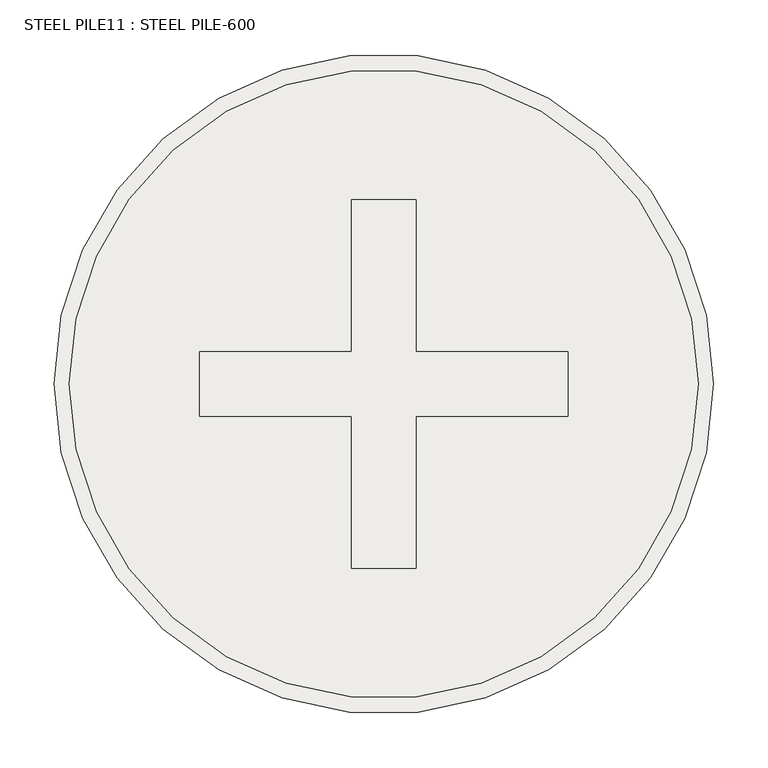
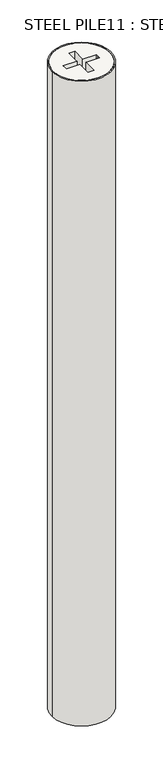
"""IFC4 building model written with IfcOpenShell, lengths in millimetres: slab geometry, STEEL PILE11 : STEEL PILE-600."""

from ifc_helpers import new_model, si_unit, point, frame, frame_2d, origin, place, context, project, spatial, circle_curve, trimmed, segment, composite_curve, outline, extrude, source, transform, mapped, element, save
from ifc_brep_helpers import plane_surface, cylinder_surface, advanced_brep


def steel_pile11_steel_pile_600_0914329d(model_context):
    return source(origin(), model_context, "Body", "SolidModel", [
        advanced_brep(
        [(5709.5, 25499.5208589, 150.0), (6290.5, 25499.5208589, 150.0), (5970.0, 25469.5208589, 150.0), (5830.0, 25469.5208589, 150.0), (5830.0, 25499.5208589, 150.0), (5830.0, 25529.5208589, 150.0), (5970.0, 25529.5208589, 150.0), (5970.0, 25669.5208589, 150.0), (6030.0, 25669.5208589, 150.0), (6030.0, 25529.5208589, 150.0), (6170.0, 25529.5208589, 150.0), (6170.0, 25499.5208589, 150.0), (6170.0, 25469.5208589, 150.0), (6030.0, 25469.5208589, 150.0), (6030.0, 25329.5208589, 150.0), (5970.0, 25329.5208589, 150.0), (5709.5, 25499.5208589, -1850.0), (6290.5, 25499.5208589, -1850.0), (5830.0, 25469.5208589, -160.0), (5970.0, 25469.5208589, -160.0), (5970.0, 25329.5208589, -160.0), (6030.0, 25329.5208589, -160.0), (6030.0, 25469.5208589, -160.0), (6170.0, 25469.5208589, -160.0), (6170.0, 25499.5208589, -160.0), (6170.0, 25529.5208589, -160.0), (6030.0, 25529.5208589, -160.0), (6030.0, 25669.5208589, -160.0), (5970.0, 25669.5208589, -160.0), (5970.0, 25529.5208589, -160.0), (5830.0, 25529.5208589, -160.0), (5830.0, 25499.5208589, -160.0)],
        [
            (0, 1, circle_curve(frame((6000.0, 25499.5208589, 150.0), z_axis=(0.0, 0.0, 1.0), x_axis=(1.0, 0.0, 0.0)), 290.5)),
            (1, 0, circle_curve(frame((6000.0, 25499.5208589, 150.0), z_axis=(0.0, 0.0, 1.0), x_axis=(1.0, 0.0, 0.0)), 290.5)),
            (2, 3),
            (3, 4),
            (4, 5),
            (5, 6),
            (6, 7),
            (7, 8),
            (8, 9),
            (9, 10),
            (10, 11),
            (11, 12),
            (12, 13),
            (13, 14),
            (14, 15),
            (15, 2),
            (16, 17, circle_curve(frame((6000.0, 25499.5208589, -1850.0), z_axis=(0.0, 0.0, -1.0), x_axis=(1.0, 0.0, 0.0)), 290.5)),
            (17, 16, circle_curve(frame((6000.0, 25499.5208589, -1850.0), z_axis=(0.0, 0.0, -1.0), x_axis=(1.0, 0.0, 0.0)), 290.5)),
            (0, 16),
            (17, 1),
            (18, 19),
            (19, 20),
            (20, 21),
            (21, 22),
            (22, 23),
            (23, 24),
            (24, 25),
            (25, 26),
            (26, 27),
            (27, 28),
            (28, 29),
            (29, 30),
            (30, 31),
            (31, 18),
            (18, 3),
            (2, 19),
            (15, 20),
            (14, 21),
            (13, 22),
            (12, 23),
            (11, 24),
            (10, 25),
            (9, 26),
            (8, 27),
            (7, 28),
            (6, 29),
            (5, 30),
            (4, 31),
        ],
        [
            plane_surface(frame((6290.5, 25499.5208589, 150.0), z_axis=(0.0, 0.0, 1.0), x_axis=(0.0, 1.0, 0.0))),
            plane_surface(frame((6290.5, 25499.5208589, -1850.0), z_axis=(0.0, 0.0, -1.0), x_axis=(0.0, -1.0, 0.0))),
            cylinder_surface(frame((6000.0, 25499.5208589, -1850.0), z_axis=(0.0, 0.0, 1.0), x_axis=(1.0, 0.0, 0.0)), 290.5),
            plane_surface(frame((5830.0, 25469.5208589, -160.0), z_axis=(0.0, 0.0, 1.0), x_axis=(-1.0, 0.0, 0.0))),
            plane_surface(frame((5830.0, 25469.5208589, 160.0), z_axis=(0.0, 1.0, 0.0), x_axis=(0.0, 0.0, -1.0))),
            plane_surface(frame((5970.0, 25469.5208589, 160.0), z_axis=(1.0, 0.0, 0.0), x_axis=(0.0, 0.0, -1.0))),
            plane_surface(frame((5970.0, 25329.5208589, 160.0), z_axis=(0.0, 1.0, 0.0), x_axis=(0.0, 0.0, -1.0))),
            plane_surface(frame((6030.0, 25329.5208589, 160.0), z_axis=(-1.0, 0.0, 0.0), x_axis=(0.0, 0.0, -1.0))),
            plane_surface(frame((6030.0, 25469.5208589, 160.0), z_axis=(0.0, 1.0, 0.0), x_axis=(0.0, 0.0, -1.0))),
            plane_surface(frame((6170.0, 25469.5208589, 160.0), z_axis=(-1.0, 0.0, 0.0), x_axis=(0.0, 0.0, -1.0))),
            plane_surface(frame((6170.0, 25499.5208589, 160.0), z_axis=(-1.0, 0.0, 0.0), x_axis=(0.0, 0.0, -1.0))),
            plane_surface(frame((6170.0, 25529.5208589, 160.0), z_axis=(0.0, -1.0, 0.0), x_axis=(0.0, 0.0, -1.0))),
            plane_surface(frame((6030.0, 25529.5208589, 160.0), z_axis=(-1.0, 0.0, 0.0), x_axis=(0.0, 0.0, -1.0))),
            plane_surface(frame((6030.0, 25669.5208589, 160.0), z_axis=(0.0, -1.0, 0.0), x_axis=(0.0, 0.0, -1.0))),
            plane_surface(frame((5970.0, 25669.5208589, 160.0), z_axis=(1.0, 0.0, 0.0), x_axis=(0.0, 0.0, -1.0))),
            plane_surface(frame((5970.0, 25529.5208589, 160.0), z_axis=(0.0, -1.0, 0.0), x_axis=(0.0, 0.0, -1.0))),
            plane_surface(frame((5830.0, 25529.5208589, 160.0), z_axis=(1.0, 0.0, 0.0), x_axis=(0.0, 0.0, -1.0))),
            plane_surface(frame((5830.0, 25499.5208589, 160.0), z_axis=(1.0, 0.0, 0.0), x_axis=(0.0, 0.0, -1.0))),
        ],
        [
            (0, [[1, 2], [3, 4, 5, 6, 7, 8, 9, 10, 11, 12, 13, 14, 15, 16]]),
            (1, [[17, 18]]),
            (2, [[-1, 19, -18, 20]]),
            (2, [[-2, -20, -17, -19]]),
            (3, [[21, 22, 23, 24, 25, 26, 27, 28, 29, 30, 31, 32, 33, 34]]),
            (4, [[-21, 35, -3, 36]]),
            (5, [[-22, -36, -16, 37]]),
            (6, [[-23, -37, -15, 38]]),
            (7, [[-24, -38, -14, 39]]),
            (8, [[-25, -39, -13, 40]]),
            (9, [[-26, -40, -12, 41]]),
            (10, [[-27, -41, -11, 42]]),
            (11, [[-28, -42, -10, 43]]),
            (12, [[-29, -43, -9, 44]]),
            (13, [[-30, -44, -8, 45]]),
            (14, [[-31, -45, -7, 46]]),
            (15, [[-32, -46, -6, 47]]),
            (16, [[-33, -47, -5, 48]]),
            (17, [[-34, -48, -4, -35]]),
        ],
    ),
        extrude(outline(composite_curve([segment(trimmed(circle_curve(frame_2d((6000.0, 25499.5208589)), 304.5), [point((5695.5, 25499.5208589))], [point((6304.5, 25499.5208589))], False, "CARTESIAN"), True, "CONTINUOUS"), segment(trimmed(circle_curve(frame_2d((6000.0, 25499.5208589)), 304.5), [point((6304.5, 25499.5208589))], [point((5695.5, 25499.5208589))], False, "CARTESIAN"), True, "CONTINUOUS")], self_intersect=False), holes=[composite_curve([segment(trimmed(circle_curve(frame_2d((6000.0, 25499.5208589)), 290.5), [point((5709.5, 25499.5208589))], [point((6290.5, 25499.5208589))], True, "CARTESIAN"), True, "CONTINUOUS"), segment(trimmed(circle_curve(frame_2d((6000.0, 25499.5208589)), 290.5), [point((6290.5, 25499.5208589))], [point((5709.5, 25499.5208589))], True, "CARTESIAN"), True, "CONTINUOUS")], self_intersect=False)]), frame((0.0, 0.0, -6850.0), z_axis=(0.0, 0.0, 1.0), x_axis=(1.0, 0.0, 0.0)), (0.0, 0.0, 1.0), 7000.0),
    ])


if __name__ == "__main__":
    model = new_model("IFC4")
    model_context = context("Model", 3, world=origin())
    ifc_project = project(units=[si_unit("LENGTHUNIT", "METRE", prefix="MILLI")], contexts=[model_context])
    site = spatial("IfcSite", under=ifc_project)
    building = spatial("IfcBuilding", under=site)
    placement = place(None, origin())
    steel_pile11_steel_pile_600_shape = steel_pile11_steel_pile_600_0914329d(model_context)
    element("IfcSlab", 1, ObjectType="STEEL PILE11 : STEEL PILE-600", at=placement, inside=building, context=model_context, shape_type="MappedRepresentation", body=[
        mapped(steel_pile11_steel_pile_600_shape, transform((0.0, 0.0, 0.0), x_axis=(1.0, 0.0, 0.0), y_axis=(0.0, 1.0, 0.0), z_axis=(0.0, 0.0, 1.0))),
    ])
    save(model, "model.ifc")
